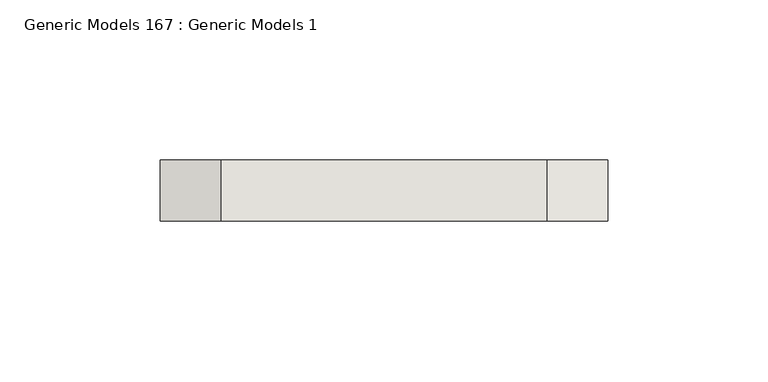
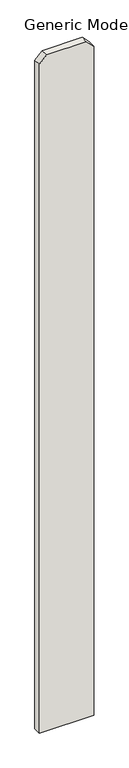
"""IFC4 building model written with IfcOpenShell, lengths in millimetres: wall geometry, Generic Models 167 : Generic Models 1."""

from ifc_helpers import new_model, si_unit, frame, origin, place, context, project, spatial, polyline, outline, extrude, source, transform, mapped, element, save


def generic_models_167_generic_models_1_61ea9d9d(model_context):
    return source(origin(), model_context, "Body", "SweptSolid", [
        extrude(outline(polyline([(76.2, 324432.6125), (1885.95, 324432.6125), (1905.0, 324413.5625), (1905.0, 324311.9625), (1885.95, 324292.9125), (76.2, 324292.9125), (76.2, 324432.6125)])), frame((0.0, 547.6875, 0.0), z_axis=(0.0, 1.0, 0.0), x_axis=(0.0, 0.0, 1.0)), (0.0, 0.0, 1.0), 19.05),
    ])


if __name__ == "__main__":
    model = new_model("IFC4")
    model_context = context("Model", 3, world=origin())
    ifc_project = project(units=[si_unit("LENGTHUNIT", "METRE", prefix="MILLI")], contexts=[model_context])
    site = spatial("IfcSite", under=ifc_project)
    building = spatial("IfcBuilding", under=site)
    placement = place(None, origin())
    generic_models_167_generic_models_1_shape = generic_models_167_generic_models_1_61ea9d9d(model_context)
    element("IfcWall", 1, ObjectType="Generic Models 167 : Generic Models 1", at=placement, inside=building, context=model_context, shape_type="MappedRepresentation", body=[
        mapped(generic_models_167_generic_models_1_shape, transform((0.0, 0.0, 0.0), x_axis=(1.0, 0.0, 0.0), y_axis=(0.0, 1.0, 0.0), z_axis=(0.0, 0.0, 1.0))),
    ])
    save(model, "model.ifc")

# Revit data of these elements
# Element 1 (IfcWall, "Generic Models 167 : Generic Models 1")
#   Materials on its faces: "VERTICAL 1X6 CEDAR PLANKS W/ CLEAR WOOD SEALER"
# Materials
#   "VERTICAL 1X6 CEDAR PLANKS W/ CLEAR WOOD SEALER": class "Wood", colour RGB 234 198 147, transparency 0, Description = "Pinus Echinata", Cost = 0
